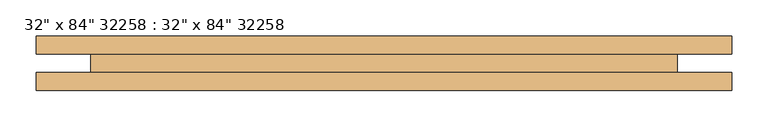
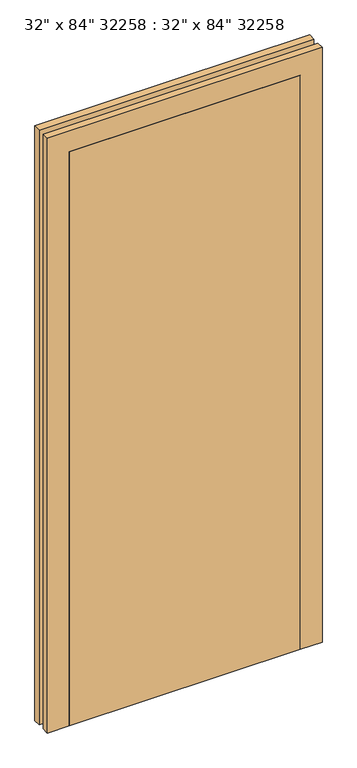
"""IFC4 building model written with IfcOpenShell, lengths in millimetres: door geometry."""

from ifc_helpers import new_model, si_unit, frame, origin, origin_with_axes, place, context, project, spatial, polyline, outline, extrude, source, transform, mapped, element, save


def door_cd82db6e(model_context):
    return source(origin(), model_context, "Body", "SweptSolid", [
        extrude(outline(polyline([(2209.8, 482.6), (2209.8, -482.6), (0.0, -482.6), (0.0, -406.4), (2133.6, -406.4), (2133.6, 406.4), (0.0, 406.4), (0.0, 482.6), (2209.8, 482.6)])), frame((0.0, 12.7, 0.0), z_axis=(0.0, 1.0, 0.0), x_axis=(0.0, 0.0, 1.0)), (0.0, 0.0, 1.0), 25.4),
        extrude(outline(polyline([(2209.8, -482.6), (0.0, -482.6), (0.0, -406.4), (2133.6, -406.4), (2133.6, 406.4), (0.0, 406.4), (0.0, 482.6), (2209.8, 482.6), (2209.8, -482.6)])), frame((0.0, -38.1, 0.0), z_axis=(0.0, 1.0, 0.0), x_axis=(0.0, 0.0, 1.0)), (0.0, 0.0, 1.0), 25.4),
        extrude(outline(polyline([(406.4, 12.7), (406.4, -38.1), (-406.4, -38.1), (-406.4, 12.7), (406.4, 12.7)])), origin_with_axes(), (0.0, 0.0, 1.0), 2133.6),
    ])


if __name__ == "__main__":
    model = new_model("IFC4")
    model_context = context("Model", 3, world=origin())
    ifc_project = project(units=[si_unit("LENGTHUNIT", "METRE", prefix="MILLI")], contexts=[model_context])
    site = spatial("IfcSite", under=ifc_project)
    building = spatial("IfcBuilding", under=site)
    placement = place(None, origin())
    door_shape = door_cd82db6e(model_context)
    element("IfcDoor", 1, ObjectType="32\" x 84\" 32258 : 32\" x 84\" 32258", at=placement, inside=building, context=model_context, shape_type="MappedRepresentation", body=[
        mapped(door_shape, transform((0.0, 0.0, 0.0), x_axis=(1.0, 0.0, 0.0), y_axis=(0.0, 1.0, 0.0), z_axis=(0.0, 0.0, 1.0))),
    ])
    save(model, "model.ifc")

# Revit data of these elements
# Type "32\" x 84\" 32258 : 32\" x 84\" 32258"
#   Type IfcGUID = "0MuvbwA9n44vt4gtWSRz0b"
#   Type Mark = "9"
#   Operation = "SINGLE_SWING_LEFT"
#   NameOverride = "32\" x 84\" 32258:32\" x 84\" 32258:302000"
#   ObjectTypeOverride = "32\" x 84\" 32258"
#   Tag = "302000"
#   Reference = "32\" x 84\""
#   ThermalTransmittance = 3.7021 (stored number, unit not read)
#   IsExternal = no
